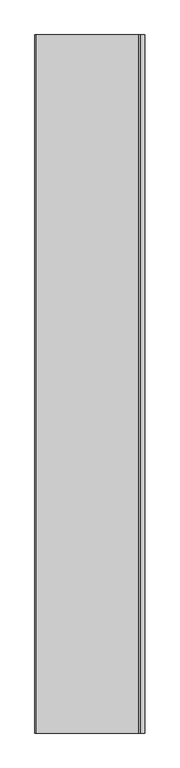
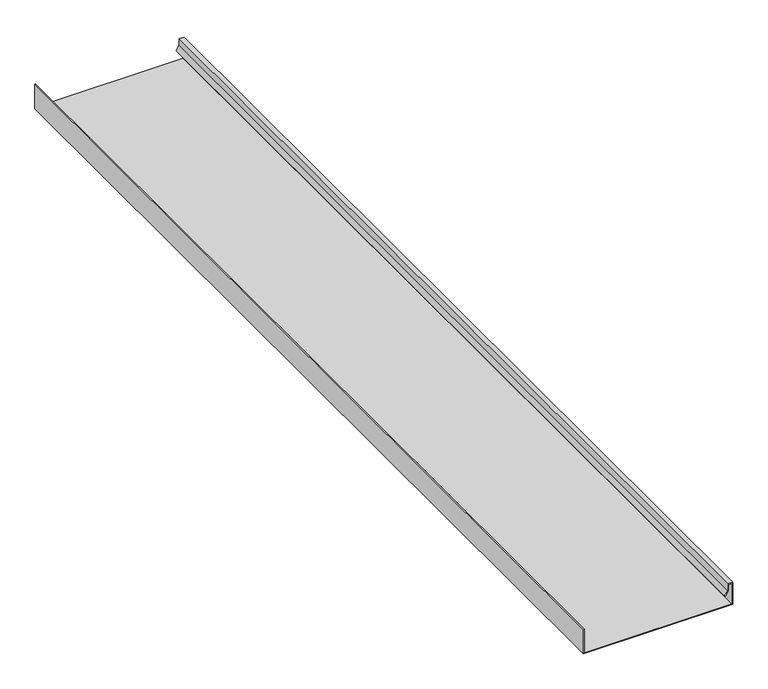
"""IFC4 building model written with IfcOpenShell, lengths in millimetres: proxy geometry, Roof001 3884 : Roof001 3884."""

from ifc_helpers import new_model, si_unit, frame, origin, place, context, project, spatial, polyline, outline, extrude, source, transform, mapped, element, save


def generic_models_ce6c4c0e(model_context):
    return source(origin(), model_context, "Body", "SweptSolid", [
        extrude(outline(polyline([(42566.0875573, -2118.238197), (42579.5727135, -2118.238197), (42579.5727135, -2111.5633924), (42534.755526, -2111.5633924), (42534.755526, -2421.9974744), (42586.5289635, -2421.9974744), (42586.5289635, -2423.9974744), (42532.755526, -2423.9974744), (42532.755526, -2109.5633924), (42581.5727135, -2109.5633924), (42581.5727135, -2120.238197), (42566.7366116, -2120.238197), (42557.4533846, -2126.9727882), (42556.2789635, -2125.3539197), (42566.0875573, -2118.238197)])), frame((0.0, -1052.8906574, 0.0), z_axis=(0.0, 1.0, 0.0), x_axis=(0.0, 0.0, 1.0)), (0.0, 0.0, 1.0), 2000.0),
    ])


if __name__ == "__main__":
    model = new_model("IFC4")
    model_context = context("Model", 3, world=origin())
    ifc_project = project(units=[si_unit("LENGTHUNIT", "METRE", prefix="MILLI")], contexts=[model_context])
    site = spatial("IfcSite", under=ifc_project)
    building = spatial("IfcBuilding", under=site)
    placement = place(None, origin())
    generic_models_shape = generic_models_ce6c4c0e(model_context)
    element("IfcBuildingElementProxy", 1, Name="Roof001 3884 : Roof001 3884", ObjectType="Roof001 3884 : Roof001 3884", at=placement, inside=building, context=model_context, shape_type="MappedRepresentation", body=[
        mapped(generic_models_shape, transform((0.0, 0.0, 0.0), x_axis=(1.0, 0.0, 0.0), y_axis=(0.0, 1.0, 0.0), z_axis=(0.0, 0.0, 1.0))),
    ])
    save(model, "model.ifc")

# Revit data of these elements
# Type "Roof001 3884 : Roof001 3884"
#   NameOverride = "Roof001"
# Element 1 (IfcBuildingElementProxy, "Roof001 3884 : Roof001 3884")
#   Materials on its faces: "STANDING SEAM METAL ROOF"
# Materials
#   "STANDING SEAM METAL ROOF": class "Unassigned", colour RGB 128 128 128, transparency 0
